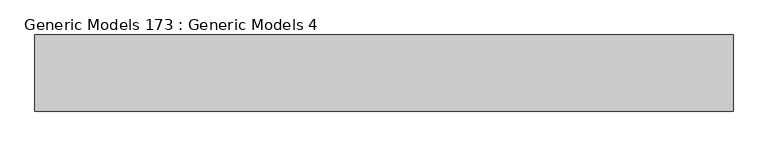
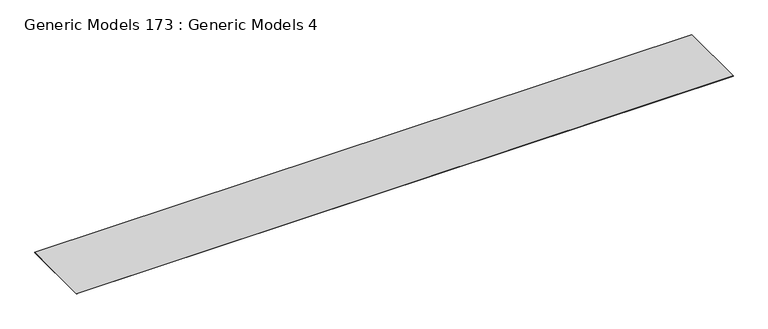
"""IFC4 building model written with IfcOpenShell, lengths in millimetres: proxy geometry, Generic Models 173 : Generic Models 4."""

import ifcopenshell
import ifcopenshell.guid

model = None  # the IFC model being written
_history = None  # IfcOwnerHistory: only IFC2X3 demands one
_inside = {}  # id of a spatial element -> (the spatial element, [elements in it])
_under = {}  # id of a project, library or spatial element -> (it, [spatial elements below it])
_declared = {}  # id of a project -> (the project, [libraries it declares])
_typed = {}  # id of a type object -> (the type object, [elements of that type])
_made_of = {}  # id of a material, layer set ... -> (it, [elements and type objects made of it])


def new_model(schema):
    """Start an empty IFC model of exactly this schema.

    Asked for "IFC4X3", IfcOpenShell would pick the latest addendum, in which some entities
    have other attributes; the version numbers below select the first issue.
    IFC2X3 requires an IfcOwnerHistory on every rooted entity: one is made here for all.
    """
    global model, _history
    if schema == "IFC4X3":
        model = ifcopenshell.file(schema_version=(4, 3, 0, 0))
    else:
        model = ifcopenshell.file(schema=schema)
    _inside.clear()
    _under.clear()
    _declared.clear()
    _typed.clear()
    _made_of.clear()
    _history = None
    if model.schema == "IFC2X3":
        org = make("IfcOrganization", Name="unknown")
        user = make(
            "IfcPersonAndOrganization",
            ThePerson=make("IfcPerson", FamilyName="unknown"),
            TheOrganization=org,
        )
        app = make(
            "IfcApplication",
            ApplicationDeveloper=org,
            Version="unknown",
            ApplicationFullName="unknown",
            ApplicationIdentifier="unknown",
        )
        _history = make(
            "IfcOwnerHistory",
            OwningUser=user,
            OwningApplication=app,
            ChangeAction="ADDED",
            CreationDate=0,
        )
    return model


def make(cls, **values):
    """One entity of the class cls with the attributes given. An attribute that is None is left unset."""
    return model.create_entity(
        cls, **{name: value for name, value in values.items() if value is not None}
    )


def rooted(cls, **values):
    """An entity with a GlobalId (a new one), such as an element, a storey or a relation."""
    return make(cls, GlobalId=ifcopenshell.guid.new(), OwnerHistory=_history, **values)


def si_unit(unit_type, name, prefix=None):
    """IfcSIUnit, for example si_unit("LENGTHUNIT", "METRE", prefix="MILLI")."""
    return make("IfcSIUnit", UnitType=unit_type, Prefix=prefix, Name=name)


def assignment(units):
    """IfcUnitAssignment: the units of a project."""
    return None if units is None else make("IfcUnitAssignment", Units=units)


def point(xyz):
    """IfcCartesianPoint."""
    return None if xyz is None else make("IfcCartesianPoint", Coordinates=xyz)


def direction(xyz):
    """IfcDirection."""
    return None if xyz is None else make("IfcDirection", DirectionRatios=xyz)


def frame(location, z_axis=None, x_axis=None):
    """IfcAxis2Placement3D, a coordinate frame: its origin and axes. An axis left out is left unset."""
    return make(
        "IfcAxis2Placement3D",
        Location=point(location),
        Axis=direction(z_axis),
        RefDirection=direction(x_axis),
    )


def origin():
    """The frame at (0, 0, 0) with its axes left unset."""
    return frame((0.0, 0.0, 0.0))


def place(relative_to, where):
    """IfcLocalPlacement: puts the frame where relative to a parent placement (None: the world)."""
    return make(
        "IfcLocalPlacement", PlacementRelTo=relative_to, RelativePlacement=where
    )


def context(
    kind, dimensions, precision=None, world=None, true_north=None, identifier=None
):
    """IfcGeometricRepresentationContext, for example the 3D "Model" context."""
    return make(
        "IfcGeometricRepresentationContext",
        ContextIdentifier=identifier,
        ContextType=kind,
        CoordinateSpaceDimension=dimensions,
        Precision=precision,
        WorldCoordinateSystem=world,
        TrueNorth=true_north,
    )


def project(units=None, contexts=None):
    """IfcProject with its units and contexts."""
    return rooted(
        "IfcProject",
        Name="project",
        RepresentationContexts=contexts,
        UnitsInContext=assignment(units),
    )


def spatial(cls, under=None, at=None, **own):
    """A site, building, storey or space (cls), placed at a placement, below another one or the project."""
    s = rooted(cls, ObjectPlacement=at, **own)
    if under is not None:
        _under.setdefault(under.id(), (under, []))[1].append(s)
    return s


def polyline(points):
    """IfcPolyline through the points."""
    return make("IfcPolyline", Points=[point(p) for p in points])


def outline(outer, holes=None, kind="AREA"):
    """IfcArbitraryClosedProfileDef: a profile drawn as a closed curve; with holes, ...WithVoids."""
    if holes is None:
        return make("IfcArbitraryClosedProfileDef", ProfileType=kind, OuterCurve=outer)
    return make(
        "IfcArbitraryProfileDefWithVoids",
        ProfileType=kind,
        OuterCurve=outer,
        InnerCurves=holes,
    )


def extrude(swept, where, along, depth):
    """IfcExtrudedAreaSolid: the profile swept, set in the frame where, extruded along a direction by depth."""
    return make(
        "IfcExtrudedAreaSolid",
        SweptArea=swept,
        Position=where,
        ExtrudedDirection=direction(along),
        Depth=depth,
    )


def shape(context_of_items, identifier, shape_type, items):
    """IfcShapeRepresentation: the items that make up one representation, for example the "Body"."""
    return make(
        "IfcShapeRepresentation",
        ContextOfItems=context_of_items,
        RepresentationIdentifier=identifier,
        RepresentationType=shape_type,
        Items=items,
    )


def source(mapping_origin, context_of_items, identifier, shape_type, items):
    """IfcRepresentationMap: a shape defined once, which mapped items show again and again."""
    return make(
        "IfcRepresentationMap",
        MappingOrigin=mapping_origin,
        MappedRepresentation=shape(context_of_items, identifier, shape_type, items),
    )


def transform(
    local_origin,
    x_axis=None,
    y_axis=None,
    z_axis=None,
    scale=None,
    scale2=None,
    scale3=None,
    uniform=True,
):
    """IfcCartesianTransformationOperator3D, or its non-uniform kind. x_axis, y_axis, z_axis: its Axis1, 2, 3."""
    if uniform:
        return make(
            "IfcCartesianTransformationOperator3D",
            Axis1=direction(x_axis),
            Axis2=direction(y_axis),
            LocalOrigin=point(local_origin),
            Scale=scale,
            Axis3=direction(z_axis),
        )
    return make(
        "IfcCartesianTransformationOperator3DnonUniform",
        Axis1=direction(x_axis),
        Axis2=direction(y_axis),
        LocalOrigin=point(local_origin),
        Scale=scale,
        Axis3=direction(z_axis),
        Scale2=scale2,
        Scale3=scale3,
    )


def mapped(mapping_source, mapping_target):
    """IfcMappedItem: shows the shape of a source again, moved by a transform."""
    return make(
        "IfcMappedItem", MappingSource=mapping_source, MappingTarget=mapping_target
    )


def made_of(thing, what):
    """Note that an element or type object is made of a material, layer set ...; save() writes the relation."""
    if what is not None:
        _made_of.setdefault(what.id(), (what, []))[1].append(thing)
    return thing


def element(
    cls,
    number,
    at=None,
    inside=None,
    cuts=None,
    type_object=None,
    material=None,
    context=None,
    identifier="Body",
    shape_type=None,
    held_by="IfcProductDefinitionShape",
    body=None,
    shapes=None,
    **own,
):
    """One element of the class cls, such as IfcWall. Its Tag is "e" and its number.

    at: its placement. inside: the storey or other place that contains it. cuts: it is an
    opening in that element (IfcRelVoidsElement). A single representation is given by context,
    identifier, shape_type and body (its items); several are given by shapes. held_by: the class
    of the entity that holds the representations. save() writes the other relations.
    """
    e = rooted(cls, Tag="e%d" % number, ObjectPlacement=at, **own)
    if body is not None:
        shapes = [shape(context, identifier, shape_type, body)]
    if shapes is not None:
        e.Representation = make(held_by, Representations=shapes)
    if inside is not None:
        _inside.setdefault(inside.id(), (inside, []))[1].append(e)
    if cuts is not None:
        rooted(
            "IfcRelVoidsElement", RelatingBuildingElement=cuts, RelatedOpeningElement=e
        )
    if type_object is not None:
        _typed.setdefault(type_object.id(), (type_object, []))[1].append(e)
    return made_of(e, material)


def aggregate(whole, parts):
    """IfcRelAggregates: a whole, such as a stair, and the parts it consists of."""
    return rooted("IfcRelAggregates", RelatingObject=whole, RelatedObjects=parts)


def save(model, path):
    """Write the relations noted so far, then the file.

    IfcRelAggregates (storeys below a building ...), IfcRelContainedInSpatialStructure (elements
    in a storey), IfcRelDefinesByType, IfcRelAssociatesMaterial and IfcRelDeclares: one each for
    every whole, place, type object, material and project.
    """
    for whole, parts in _under.values():
        aggregate(whole, parts)
    for where, things in _inside.values():
        rooted(
            "IfcRelContainedInSpatialStructure",
            RelatedElements=things,
            RelatingStructure=where,
        )
    for kind, things in _typed.values():
        rooted("IfcRelDefinesByType", RelatedObjects=things, RelatingType=kind)
    for what, things in _made_of.values():
        rooted("IfcRelAssociatesMaterial", RelatedObjects=things, RelatingMaterial=what)
    for by, libraries in _declared.values():
        rooted("IfcRelDeclares", RelatingContext=by, RelatedDefinitions=libraries)
    model.write(path)


def generic_models_173_generic_models_4_f253a565(model_context):
    return source(origin(), model_context, "Body", "SweptSolid", [
        extrude(outline(polyline([(28171.2958007, -7352.2318256), (28171.2958007, -7897.898997), (23168.0573109, -7897.898997), (23168.0573109, -7352.2318256), (28171.2958007, -7352.2318256)])), frame((0.0, 0.0, 123156.4085), z_axis=(0.0, 0.0, 1.0), x_axis=(1.0, 0.0, 0.0)), (0.0, 0.0, 1.0), 1.5875),
    ])


if __name__ == "__main__":
    model = new_model("IFC4")
    model_context = context("Model", 3, world=origin())
    ifc_project = project(units=[si_unit("LENGTHUNIT", "METRE", prefix="MILLI")], contexts=[model_context])
    site = spatial("IfcSite", under=ifc_project)
    building = spatial("IfcBuilding", under=site)
    placement = place(None, origin())
    generic_models_173_generic_models_4_shape = generic_models_173_generic_models_4_f253a565(model_context)
    element("IfcBuildingElementProxy", 1, Name="Generic Models 173 : Generic Models 4", ObjectType="Generic Models 173 : Generic Models 4", at=placement, inside=building, context=model_context, shape_type="MappedRepresentation", body=[
        mapped(generic_models_173_generic_models_4_shape, transform((0.0, 0.0, 0.0), x_axis=(1.0, 0.0, 0.0), y_axis=(0.0, 1.0, 0.0), z_axis=(0.0, 0.0, 1.0))),
    ])
    save(model, "model.ifc")

# Revit data of these elements
# Element 1 (IfcBuildingElementProxy, "Generic Models 173 : Generic Models 4")
#   Materials on its faces: "_15 MIL VAPOR BARRIER"
# Materials
#   "_15 MIL VAPOR BARRIER": class "Generic", colour RGB 67 154 161, transparency 0, Cost = 0
